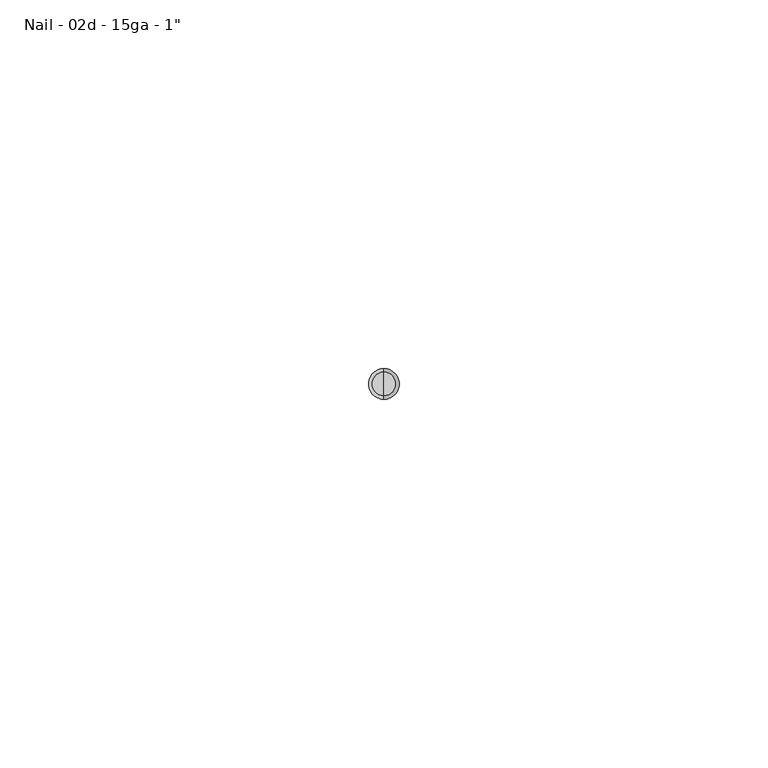
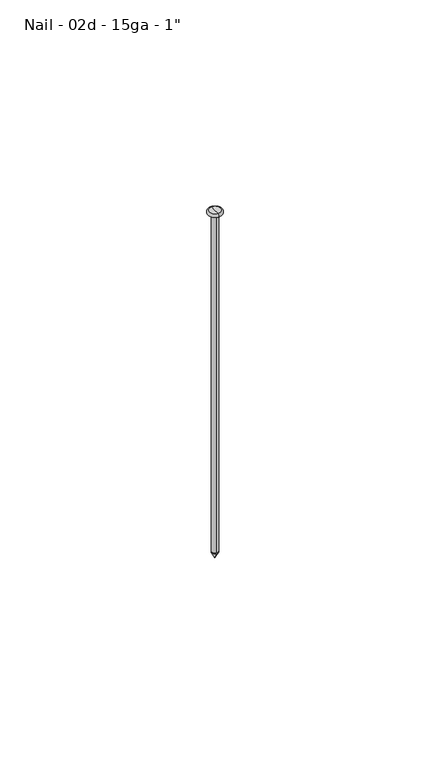
"""IFC4 building model written with IfcOpenShell, lengths in millimetres: fastener geometry."""

from ifc_helpers import new_model, si_unit, point, frame, origin, origin_2d, place, context, project, spatial, polyline, circle_curve, ellipse_curve, trimmed, segment, composite_curve, outline, extrude, source, transform, mapped, element, save
from ifc_brep_helpers import plane_surface, revolved_surface, advanced_brep


def fastener_8ce62b08(model_context):
    return source(origin(), model_context, "Body", "SolidModel", [
        advanced_brep(
        [(0.0, -0.9144, -101.6), (0.0, 0.9144, -101.6), (0.0, 0.0, -101.6), (0.0, 0.0, -103.4288)],
        [
            (0, 1, circle_curve(frame((0.0, 0.0, -101.6), z_axis=(0.0, 0.0, 1.0), x_axis=(0.0, 1.0, 0.0)), 0.9144)),
            (1, 2),
            (2, 0),
            (1, 0, circle_curve(frame((0.0, 0.0, -101.6), z_axis=(0.0, 0.0, 1.0), x_axis=(0.0, 1.0, 0.0)), 0.9144)),
            (3, 1),
            (0, 3),
        ],
        [
            plane_surface(frame((0.0, 0.0, -101.6), z_axis=(0.0, 0.0, 1.0), x_axis=(0.0, 1.0, 0.0))),
            revolved_surface(polyline([(0.0, 0.9144, -101.6), (0.0, 0.0, -103.4288)]), (0.0, 0.0, -103.0840259), (0.0, 0.0, -1.0)),
        ],
        [
            (0, [[1, 2, 3]]),
            (0, [[4, -3, -2]]),
            (1, [[5, -1, 6]]),
            (1, [[-6, -4, -5]]),
        ],
    ),
        advanced_brep(
        [(0.0, 1.8288, 0.0), (0.0, -1.8288, 0.0), (0.0, 0.0, 0.0), (0.0, 0.0, 0.9144), (0.0, -1.5875, 0.9144), (0.0, 1.5875, 0.9144)],
        [
            (0, 1, circle_curve(frame((0.0, 0.0, 0.0), z_axis=(0.0, 0.0, -1.0), x_axis=(0.0, -1.0, 0.0)), 1.8288)),
            (1, 2),
            (2, 0),
            (1, 0, circle_curve(frame((0.0, 0.0, 0.0), z_axis=(0.0, 0.0, -1.0), x_axis=(0.0, -1.0, 0.0)), 1.8288)),
            (3, 4),
            (4, 5, circle_curve(frame((0.0, 0.0, 0.9144), z_axis=(0.0, 0.0, 1.0), x_axis=(0.0, -1.0, 0.0)), 1.5875)),
            (5, 3),
            (5, 4, circle_curve(frame((0.0, 0.0, 0.9144), z_axis=(0.0, 0.0, 1.0), x_axis=(0.0, -1.0, 0.0)), 1.5875)),
            (4, 1, circle_curve(frame((0.0, -1.5875, 0.4253618), z_axis=(1.0, 0.0, 0.0), x_axis=(0.0, -1.0, 0.0)), 0.4890382)),
            (0, 5, circle_curve(frame((0.0, 1.5875, 0.4253618), z_axis=(1.0, 0.0, 0.0), x_axis=(0.0, 1.0, 0.0)), 0.4890382)),
        ],
        [
            plane_surface(frame((0.0, 0.0, 0.0), z_axis=(0.0, 0.0, -1.0), x_axis=(0.0, -1.0, 0.0))),
            plane_surface(frame((0.0, 0.0, 0.9144), z_axis=(0.0, 0.0, 1.0), x_axis=(0.0, -1.0, 0.0))),
            revolved_surface(trimmed(ellipse_curve(frame((0.0, -1.5875, 0.4253618), z_axis=(-1.0, 0.0, 0.0), x_axis=(0.0, -1.0, 0.0)), 0.4890382, 0.4890382), [point((0.0, -1.8288, 0.0))], [point((0.0, -1.5875, 0.9144))], True, "CARTESIAN"), (0.0, 0.0, 1.4840259), (0.0, 0.0, 1.0)),
        ],
        [
            (0, [[1, 2, 3]]),
            (0, [[4, -3, -2]]),
            (1, [[5, 6, 7]]),
            (1, [[-7, 8, -5]]),
            (2, [[-6, 9, -1, 10]]),
            (2, [[-8, -10, -4, -9]]),
        ],
    ),
        extrude(outline(composite_curve([segment(trimmed(circle_curve(origin_2d(), 0.9144), [point((0.0, -0.9144))], [point((0.0, 0.9144))], False, "CARTESIAN"), True, "CONTINUOUS"), segment(trimmed(circle_curve(origin_2d(), 0.9144), [point((0.0, 0.9144))], [point((0.0, -0.9144))], False, "CARTESIAN"), True, "CONTINUOUS")], self_intersect=False)), frame((0.0, 0.0, -101.6), z_axis=(0.0, 0.0, 1.0), x_axis=(1.0, 0.0, 0.0)), (0.0, 0.0, 1.0), 101.6),
    ])


if __name__ == "__main__":
    model = new_model("IFC4")
    model_context = context("Model", 3, world=origin())
    ifc_project = project(units=[si_unit("LENGTHUNIT", "METRE", prefix="MILLI")], contexts=[model_context])
    site = spatial("IfcSite", under=ifc_project)
    building = spatial("IfcBuilding", under=site)
    placement = place(None, origin())
    fastener_shape = fastener_8ce62b08(model_context)
    element("IfcFastener", 1, ObjectType="060523 - W_P_C - Fastenings - Generic : Nail - 02d - 15ga - 1\"", at=placement, inside=building, context=model_context, shape_type="MappedRepresentation", body=[
        mapped(fastener_shape, transform((0.0, 0.0, 0.0), x_axis=(1.0, 0.0, 0.0), y_axis=(0.0, 1.0, 0.0), z_axis=(0.0, 0.0, 1.0))),
    ])
    save(model, "model.ifc")

# Revit data of these elements
# Type "060523 - W_P_C - Fastenings - Generic : Nail - 02d - 15ga - 1\""
#   Washer_Thickness = 0' - 0.00333"
#   Washer Radius = 0' - 0.046"
#   Washer Offset - Head = 0' - 0"
#   Washer Offset = 0' - 0"
#   Thickness_of_Substrate [instance default] = 0' - 1"
#   Side = 0' - 0 37/64"
#   Radius = 0' - 0.036"
#   Length [instance default] = 0' - 1"
#   Head Size = 0' - 1"
#   Head Radius = 0' - 0 1/2"
#   Head Height = 0' - 0.01"
#   Double Diameter = 0' - 0.144"
#   Diameter = 0' - 0.072"
#   Default Elevation = 4' - 0"
#   Washer_Nut_Visibility = no
#   Washer_Head_Visibility = no
#   Round_Head_Visibility = yes
#   Point Visibility = yes
#   Nut_Visibility = no
#   Hex_Head_Visiblilty = no
#   Washer Material = none
#   Bolt Material (Size) = AT SILL - FASTENER AT 24" O.C.
# Element 1 (IfcFastener, "060523 - W_P_C - Fastenings - Generic : Nail - 02d - 15ga - 1\"")
#   Length = 0' - 4"
#   Materials on its faces: "AT SILL - FASTENER AT 24\" O.C."
# Materials
#   "AT SILL - FASTENER AT 24\" O.C.": class "Generic", colour RGB 120 120 120, transparency 0, Cost = 0
